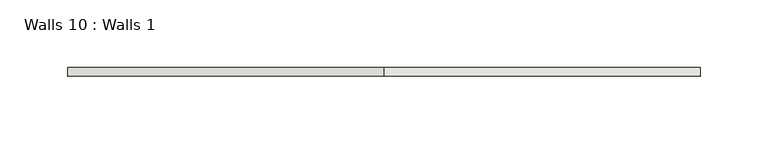
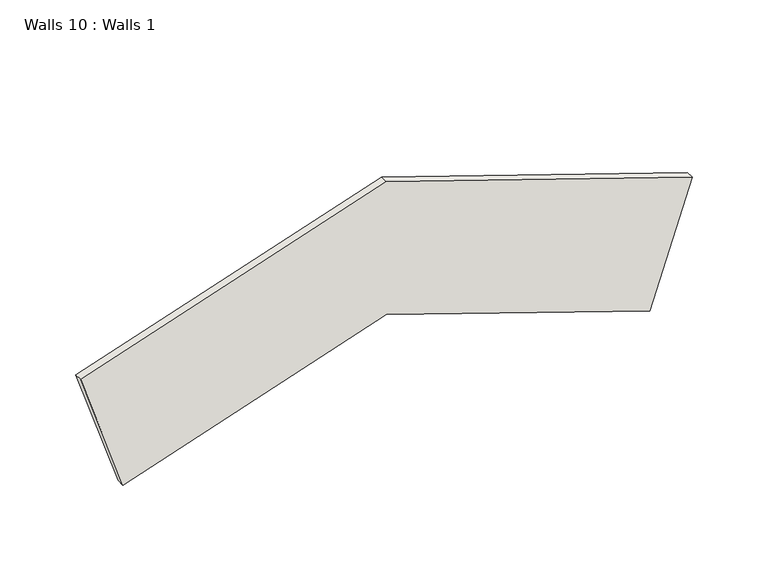
"""IFC4 building model written with IfcOpenShell, lengths in millimetres: wall geometry, Walls 10 : Walls 1."""

from ifc_helpers import new_model, si_unit, frame, origin, place, context, project, spatial, polyline, outline, extrude, source, transform, mapped, element, save


def walls_10_walls_1_c91e7d2d(model_context):
    return source(origin(), model_context, "Body", "SweptSolid", [
        extrude(outline(polyline([(5458.0690223, 21244.0906427), (5525.2438111, 21444.7370052), (5458.0690223, 21645.3833677), (5554.4130034, 21677.6385579), (5632.3865706, 21444.7370052), (5554.4130034, 21211.8354525), (5458.0690223, 21244.0906427)])), frame((0.0, -1122.6884634, 0.0), z_axis=(0.0, 1.0, 0.0), x_axis=(0.0, 0.0, 1.0)), (0.0, 0.0, 1.0), 6.35),
    ])


if __name__ == "__main__":
    model = new_model("IFC4")
    model_context = context("Model", 3, world=origin())
    ifc_project = project(units=[si_unit("LENGTHUNIT", "METRE", prefix="MILLI")], contexts=[model_context])
    site = spatial("IfcSite", under=ifc_project)
    building = spatial("IfcBuilding", under=site)
    placement = place(None, origin())
    walls_10_walls_1_shape = walls_10_walls_1_c91e7d2d(model_context)
    element("IfcWall", 1, ObjectType="Walls 10 : Walls 1", at=placement, inside=building, context=model_context, shape_type="MappedRepresentation", body=[
        mapped(walls_10_walls_1_shape, transform((0.0, 0.0, 0.0), x_axis=(1.0, 0.0, 0.0), y_axis=(0.0, 1.0, 0.0), z_axis=(0.0, 0.0, 1.0))),
    ])
    save(model, "model.ifc")

# Revit data of these elements
# Element 1 (IfcWall, "Walls 10 : Walls 1")
#   Materials on its faces: "1/4\" STEEL GUSSET PLATE - (RAW STEEL)"
# Materials
#   "1/4\" STEEL GUSSET PLATE - (RAW STEEL)": class "Metal", colour RGB 189 187 185, transparency 0, Description = "Structural steel 50ksi", Cost = 0
